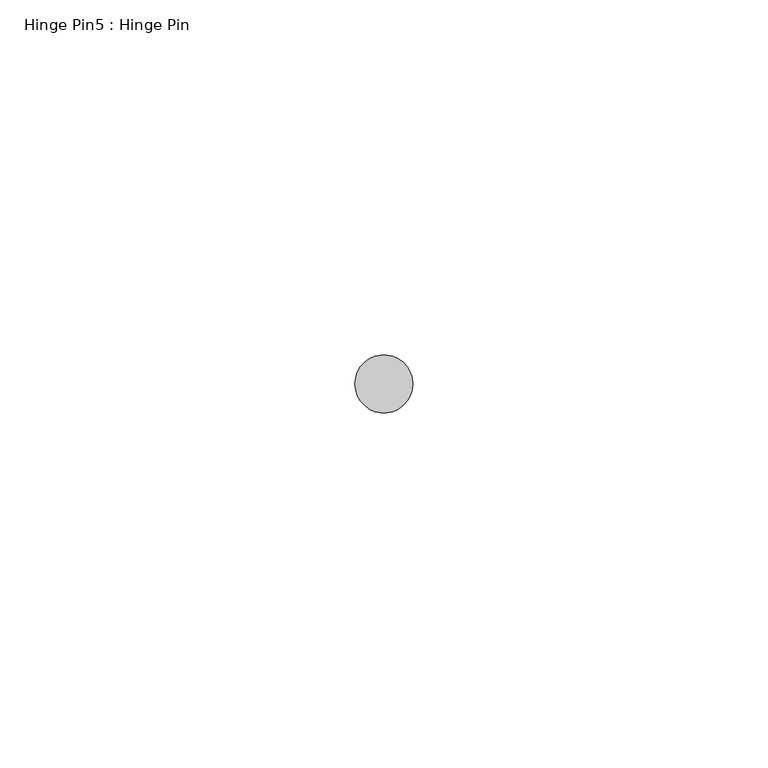
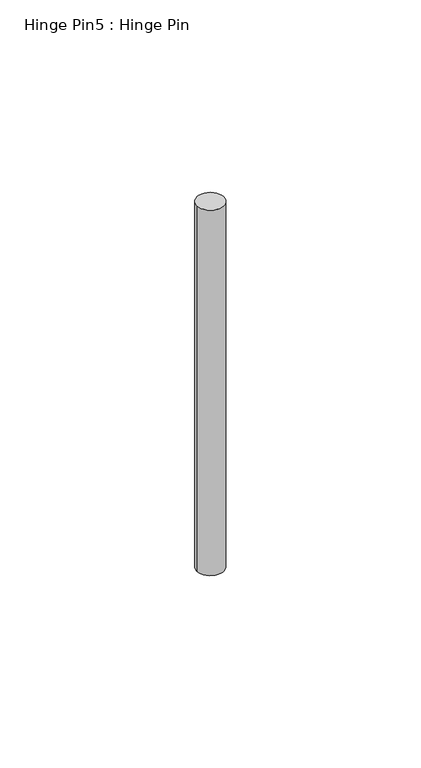
"""IFC4 building model written with IfcOpenShell, lengths in millimetres: proxy geometry, Hinge Pin5 : Hinge Pin."""

from ifc_helpers import new_model, si_unit, point, frame, frame_2d, origin, place, context, project, spatial, circle_curve, trimmed, segment, composite_curve, outline, extrude, source, transform, mapped, element, save


def hinge_pin5_hinge_pin_e8284dc3(model_context):
    return source(origin(), model_context, "Body", "SweptSolid", [
        extrude(outline(composite_curve([segment(trimmed(circle_curve(frame_2d((587319.1320739, -533984.6777841)), 4.0894), [point((587315.0426739, -533984.6777841))], [point((587323.2214739, -533984.6777841))], False, "CARTESIAN"), True, "CONTINUOUS"), segment(trimmed(circle_curve(frame_2d((587319.1320739, -533984.6777841)), 4.0894), [point((587323.2214739, -533984.6777841))], [point((587315.0426739, -533984.6777841))], False, "CARTESIAN"), True, "CONTINUOUS")], self_intersect=False)), frame((0.0, 0.0, 1128.5140625), z_axis=(0.0, 0.0, 1.0), x_axis=(1.0, 0.0, 0.0)), (0.0, 0.0, 1.0), 117.871875),
    ])


if __name__ == "__main__":
    model = new_model("IFC4")
    model_context = context("Model", 3, world=origin())
    ifc_project = project(units=[si_unit("LENGTHUNIT", "METRE", prefix="MILLI")], contexts=[model_context])
    site = spatial("IfcSite", under=ifc_project)
    building = spatial("IfcBuilding", under=site)
    placement = place(None, origin())
    hinge_pin5_hinge_pin_shape = hinge_pin5_hinge_pin_e8284dc3(model_context)
    element("IfcBuildingElementProxy", 1, Name="Hinge Pin5 : Hinge Pin", ObjectType="Hinge Pin5 : Hinge Pin", at=placement, inside=building, context=model_context, shape_type="MappedRepresentation", body=[
        mapped(hinge_pin5_hinge_pin_shape, transform((0.0, 0.0, 0.0), x_axis=(1.0, 0.0, 0.0), y_axis=(0.0, 1.0, 0.0), z_axis=(0.0, 0.0, 1.0))),
    ])
    save(model, "model.ifc")

# Revit data of these elements
# Element 1 (IfcBuildingElementProxy, "Hinge Pin5 : Hinge Pin")
#   Materials on its faces: "6\"X6\" WELD-ON STL BUTT HINGE"
# Materials
#   "6\"X6\" WELD-ON STL BUTT HINGE": class "Metal", colour RGB 189 187 185, transparency 0, Description = "Carbon steel", Cost = 0
